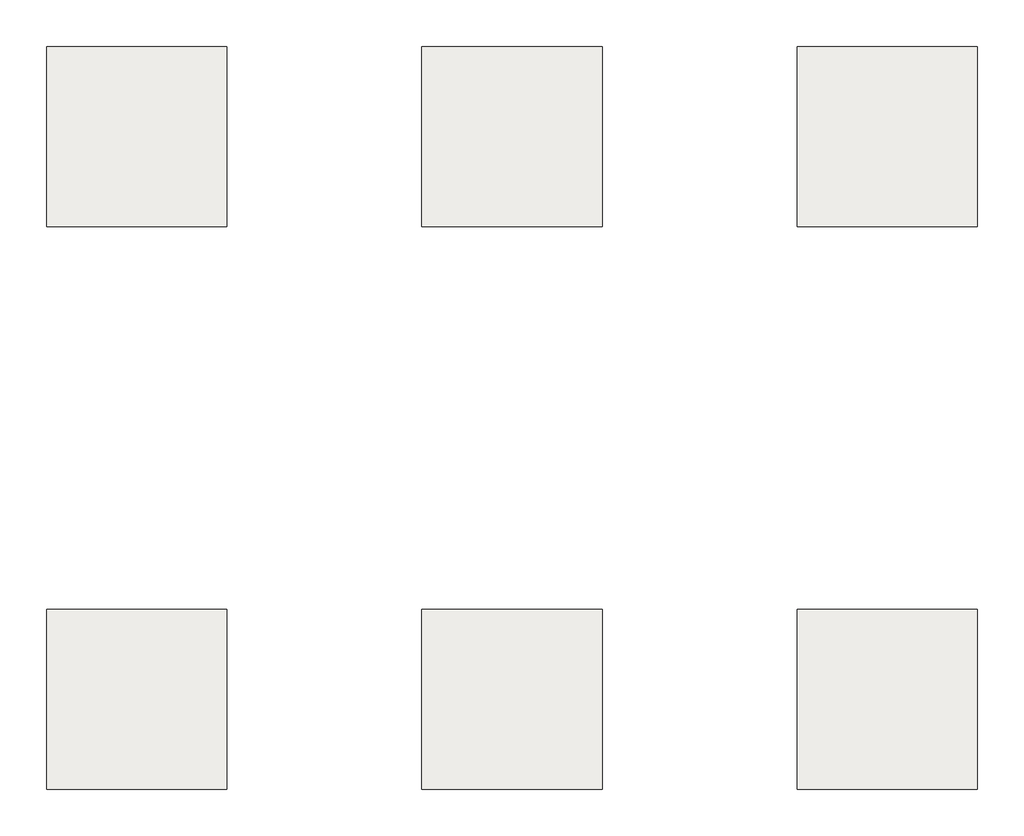
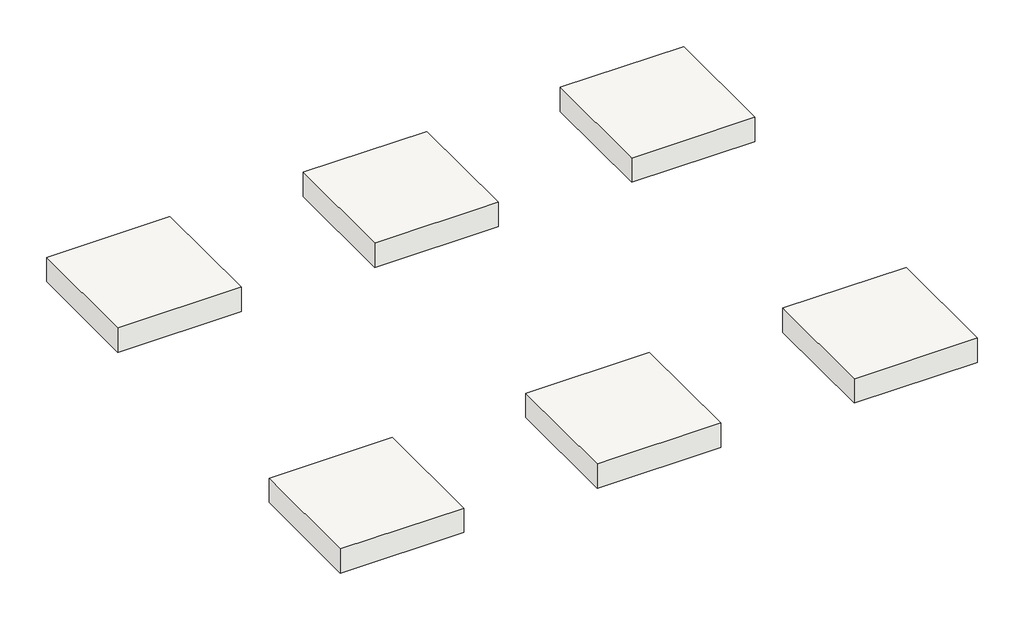
# One storey: 6 slabs.
"""IFC4 building model written with IfcOpenShell, lengths in millimetres."""

import ifcopenshell
import ifcopenshell.guid

model = None  # the IFC model being written
_history = None  # IfcOwnerHistory: only IFC2X3 demands one
_inside = {}  # id of a spatial element -> (the spatial element, [elements in it])
_under = {}  # id of a project, library or spatial element -> (it, [spatial elements below it])
_declared = {}  # id of a project -> (the project, [libraries it declares])
_typed = {}  # id of a type object -> (the type object, [elements of that type])
_made_of = {}  # id of a material, layer set ... -> (it, [elements and type objects made of it])


def new_model(schema):
    """Start an empty IFC model of exactly this schema.

    Asked for "IFC4X3", IfcOpenShell would pick the latest addendum, in which some entities
    have other attributes; the version numbers below select the first issue.
    IFC2X3 requires an IfcOwnerHistory on every rooted entity: one is made here for all.
    """
    global model, _history
    if schema == "IFC4X3":
        model = ifcopenshell.file(schema_version=(4, 3, 0, 0))
    else:
        model = ifcopenshell.file(schema=schema)
    _inside.clear()
    _under.clear()
    _declared.clear()
    _typed.clear()
    _made_of.clear()
    _history = None
    if model.schema == "IFC2X3":
        org = make("IfcOrganization", Name="unknown")
        user = make(
            "IfcPersonAndOrganization",
            ThePerson=make("IfcPerson", FamilyName="unknown"),
            TheOrganization=org,
        )
        app = make(
            "IfcApplication",
            ApplicationDeveloper=org,
            Version="unknown",
            ApplicationFullName="unknown",
            ApplicationIdentifier="unknown",
        )
        _history = make(
            "IfcOwnerHistory",
            OwningUser=user,
            OwningApplication=app,
            ChangeAction="ADDED",
            CreationDate=0,
        )
    return model


def make(cls, **values):
    """One entity of the class cls with the attributes given. An attribute that is None is left unset."""
    return model.create_entity(
        cls, **{name: value for name, value in values.items() if value is not None}
    )


def rooted(cls, **values):
    """An entity with a GlobalId (a new one), such as an element, a storey or a relation."""
    return make(cls, GlobalId=ifcopenshell.guid.new(), OwnerHistory=_history, **values)


def si_unit(unit_type, name, prefix=None):
    """IfcSIUnit, for example si_unit("LENGTHUNIT", "METRE", prefix="MILLI")."""
    return make("IfcSIUnit", UnitType=unit_type, Prefix=prefix, Name=name)


def assignment(units):
    """IfcUnitAssignment: the units of a project."""
    return None if units is None else make("IfcUnitAssignment", Units=units)


def point(xyz):
    """IfcCartesianPoint."""
    return None if xyz is None else make("IfcCartesianPoint", Coordinates=xyz)


def direction(xyz):
    """IfcDirection."""
    return None if xyz is None else make("IfcDirection", DirectionRatios=xyz)


def frame(location, z_axis=None, x_axis=None):
    """IfcAxis2Placement3D, a coordinate frame: its origin and axes. An axis left out is left unset."""
    return make(
        "IfcAxis2Placement3D",
        Location=point(location),
        Axis=direction(z_axis),
        RefDirection=direction(x_axis),
    )


def origin():
    """The frame at (0, 0, 0) with its axes left unset."""
    return frame((0.0, 0.0, 0.0))


def place(relative_to, where):
    """IfcLocalPlacement: puts the frame where relative to a parent placement (None: the world)."""
    return make(
        "IfcLocalPlacement", PlacementRelTo=relative_to, RelativePlacement=where
    )


def context(
    kind, dimensions, precision=None, world=None, true_north=None, identifier=None
):
    """IfcGeometricRepresentationContext, for example the 3D "Model" context."""
    return make(
        "IfcGeometricRepresentationContext",
        ContextIdentifier=identifier,
        ContextType=kind,
        CoordinateSpaceDimension=dimensions,
        Precision=precision,
        WorldCoordinateSystem=world,
        TrueNorth=true_north,
    )


def project(units=None, contexts=None):
    """IfcProject with its units and contexts."""
    return rooted(
        "IfcProject",
        Name="project",
        RepresentationContexts=contexts,
        UnitsInContext=assignment(units),
    )


def spatial(cls, under=None, at=None, **own):
    """A site, building, storey or space (cls), placed at a placement, below another one or the project."""
    s = rooted(cls, ObjectPlacement=at, **own)
    if under is not None:
        _under.setdefault(under.id(), (under, []))[1].append(s)
    return s


def polyline(points):
    """IfcPolyline through the points."""
    return make("IfcPolyline", Points=[point(p) for p in points])


def outline(outer, holes=None, kind="AREA"):
    """IfcArbitraryClosedProfileDef: a profile drawn as a closed curve; with holes, ...WithVoids."""
    if holes is None:
        return make("IfcArbitraryClosedProfileDef", ProfileType=kind, OuterCurve=outer)
    return make(
        "IfcArbitraryProfileDefWithVoids",
        ProfileType=kind,
        OuterCurve=outer,
        InnerCurves=holes,
    )


def extrude(swept, where, along, depth):
    """IfcExtrudedAreaSolid: the profile swept, set in the frame where, extruded along a direction by depth."""
    return make(
        "IfcExtrudedAreaSolid",
        SweptArea=swept,
        Position=where,
        ExtrudedDirection=direction(along),
        Depth=depth,
    )


def shape(context_of_items, identifier, shape_type, items):
    """IfcShapeRepresentation: the items that make up one representation, for example the "Body"."""
    return make(
        "IfcShapeRepresentation",
        ContextOfItems=context_of_items,
        RepresentationIdentifier=identifier,
        RepresentationType=shape_type,
        Items=items,
    )


def source(mapping_origin, context_of_items, identifier, shape_type, items):
    """IfcRepresentationMap: a shape defined once, which mapped items show again and again."""
    return make(
        "IfcRepresentationMap",
        MappingOrigin=mapping_origin,
        MappedRepresentation=shape(context_of_items, identifier, shape_type, items),
    )


def transform(
    local_origin,
    x_axis=None,
    y_axis=None,
    z_axis=None,
    scale=None,
    scale2=None,
    scale3=None,
    uniform=True,
):
    """IfcCartesianTransformationOperator3D, or its non-uniform kind. x_axis, y_axis, z_axis: its Axis1, 2, 3."""
    if uniform:
        return make(
            "IfcCartesianTransformationOperator3D",
            Axis1=direction(x_axis),
            Axis2=direction(y_axis),
            LocalOrigin=point(local_origin),
            Scale=scale,
            Axis3=direction(z_axis),
        )
    return make(
        "IfcCartesianTransformationOperator3DnonUniform",
        Axis1=direction(x_axis),
        Axis2=direction(y_axis),
        LocalOrigin=point(local_origin),
        Scale=scale,
        Axis3=direction(z_axis),
        Scale2=scale2,
        Scale3=scale3,
    )


def mapped(mapping_source, mapping_target):
    """IfcMappedItem: shows the shape of a source again, moved by a transform."""
    return make(
        "IfcMappedItem", MappingSource=mapping_source, MappingTarget=mapping_target
    )


def made_of(thing, what):
    """Note that an element or type object is made of a material, layer set ...; save() writes the relation."""
    if what is not None:
        _made_of.setdefault(what.id(), (what, []))[1].append(thing)
    return thing


def element(
    cls,
    number,
    at=None,
    inside=None,
    cuts=None,
    type_object=None,
    material=None,
    context=None,
    identifier="Body",
    shape_type=None,
    held_by="IfcProductDefinitionShape",
    body=None,
    shapes=None,
    **own,
):
    """One element of the class cls, such as IfcWall. Its Tag is "e" and its number.

    at: its placement. inside: the storey or other place that contains it. cuts: it is an
    opening in that element (IfcRelVoidsElement). A single representation is given by context,
    identifier, shape_type and body (its items); several are given by shapes. held_by: the class
    of the entity that holds the representations. save() writes the other relations.
    """
    e = rooted(cls, Tag="e%d" % number, ObjectPlacement=at, **own)
    if body is not None:
        shapes = [shape(context, identifier, shape_type, body)]
    if shapes is not None:
        e.Representation = make(held_by, Representations=shapes)
    if inside is not None:
        _inside.setdefault(inside.id(), (inside, []))[1].append(e)
    if cuts is not None:
        rooted(
            "IfcRelVoidsElement", RelatingBuildingElement=cuts, RelatedOpeningElement=e
        )
    if type_object is not None:
        _typed.setdefault(type_object.id(), (type_object, []))[1].append(e)
    return made_of(e, material)


def aggregate(whole, parts):
    """IfcRelAggregates: a whole, such as a stair, and the parts it consists of."""
    return rooted("IfcRelAggregates", RelatingObject=whole, RelatedObjects=parts)


def save(model, path):
    """Write the relations noted so far, then the file.

    IfcRelAggregates (storeys below a building ...), IfcRelContainedInSpatialStructure (elements
    in a storey), IfcRelDefinesByType, IfcRelAssociatesMaterial and IfcRelDeclares: one each for
    every whole, place, type object, material and project.
    """
    for whole, parts in _under.values():
        aggregate(whole, parts)
    for where, things in _inside.values():
        rooted(
            "IfcRelContainedInSpatialStructure",
            RelatedElements=things,
            RelatingStructure=where,
        )
    for kind, things in _typed.values():
        rooted("IfcRelDefinesByType", RelatedObjects=things, RelatingType=kind)
    for what, things in _made_of.values():
        rooted("IfcRelAssociatesMaterial", RelatedObjects=things, RelatingMaterial=what)
    for by, libraries in _declared.values():
        rooted("IfcRelDeclares", RelatingContext=by, RelatedDefinitions=libraries)
    model.write(path)


def ft112_footing_rectangular_ft112_2400x2400x500_5fe39465(model_context):
    return source(origin(), model_context, "Body", "SweptSolid", [
        extrude(outline(polyline([(1200.0, 1200.0), (1200.0, -1200.0), (-1200.0, -1200.0), (-1200.0, 1200.0), (1200.0, 1200.0)])), frame((0.0, 0.0, -500.0), z_axis=(0.0, 0.0, 1.0), x_axis=(1.0, 0.0, 0.0)), (0.0, 0.0, 1.0), 500.0),
    ])


model = new_model("IFC4")

# Units and contexts
model_context = context("Model", 3, world=origin())
ifc_project = project(units=[si_unit("LENGTHUNIT", "METRE", prefix="MILLI")], contexts=[model_context])

# Site, building, storey
site = spatial("IfcSite", under=ifc_project)
building = spatial("IfcBuilding", under=site)
storey = spatial("IfcBuildingStorey", under=building, Name="B.O.F", Elevation=-1800.0)

# Slabs
placement = place(None, origin())
ft112_footing_rectangular_ft112_2400x2400x500_shape = ft112_footing_rectangular_ft112_2400x2400x500_5fe39465(model_context)
element("IfcSlab", 1, ObjectType="FT112-Footing-Rectangular : FT112_2400x2400x500", at=placement, inside=storey, context=model_context, shape_type="MappedRepresentation", body=[
    mapped(ft112_footing_rectangular_ft112_2400x2400x500_shape, transform((4920.0, 13499.5208589, -1300.0), x_axis=(1.0, 0.0, 0.0), y_axis=(0.0, 1.0, 0.0), z_axis=(0.0, 0.0, 1.0))),
])
element("IfcSlab", 2, ObjectType="FT112-Footing-Rectangular : FT112_2400x2400x500", at=placement, inside=storey, context=model_context, shape_type="MappedRepresentation", body=[
    mapped(ft112_footing_rectangular_ft112_2400x2400x500_shape, transform((9920.0, 13499.5208589, -1300.0), x_axis=(1.0, 0.0, 0.0), y_axis=(0.0, 1.0, 0.0), z_axis=(0.0, 0.0, 1.0))),
])
element("IfcSlab", 3, ObjectType="FT112-Footing-Rectangular : FT112_2400x2400x500", at=placement, inside=storey, context=model_context, shape_type="MappedRepresentation", body=[
    mapped(ft112_footing_rectangular_ft112_2400x2400x500_shape, transform((9920.0, 20999.5208589, -1300.0), x_axis=(1.0, 0.0, 0.0), y_axis=(0.0, 1.0, 0.0), z_axis=(0.0, 0.0, 1.0))),
])
element("IfcSlab", 4, ObjectType="FT112-Footing-Rectangular : FT112_2400x2400x500", at=placement, inside=storey, context=model_context, shape_type="MappedRepresentation", body=[
    mapped(ft112_footing_rectangular_ft112_2400x2400x500_shape, transform((4920.0, 20999.5208589, -1300.0), x_axis=(1.0, 0.0, 0.0), y_axis=(0.0, 1.0, 0.0), z_axis=(0.0, 0.0, 1.0))),
])
element("IfcSlab", 5, ObjectType="FT112-Footing-Rectangular : FT112_2400x2400x500", at=placement, inside=storey, context=model_context, shape_type="MappedRepresentation", body=[
    mapped(ft112_footing_rectangular_ft112_2400x2400x500_shape, transform((-80.0, 20999.5208589, -1300.0), x_axis=(1.0, 0.0, 0.0), y_axis=(0.0, 1.0, 0.0), z_axis=(0.0, 0.0, 1.0))),
])
element("IfcSlab", 6, ObjectType="FT112-Footing-Rectangular : FT112_2400x2400x500", at=placement, inside=storey, context=model_context, shape_type="MappedRepresentation", body=[
    mapped(ft112_footing_rectangular_ft112_2400x2400x500_shape, transform((-80.0, 13499.5208589, -1300.0), x_axis=(1.0, 0.0, 0.0), y_axis=(0.0, 1.0, 0.0), z_axis=(0.0, 0.0, 1.0))),
])

save(model, "model.ifc")

# Revit data of these elements
# Project information
#   Building Name = "MAIN GATE SECURITY BUILDING"
#   Project Status = "Project Status"
#   Client Name = "현대엔지니어링"
#   Project Address = "서울시 종로구 율곡로 75(계동)"
#   Project Name = "Therma Visayas Energy Project"
#   Project Number = "-"
# Grids (mm)
#   "B": line (5000, 25626.165) -> (5000, 10142.075)
#   "C": line (10000, 25626.165) -> (10000, 10142.075)
#   "A": line (0, 25626.165) -> (0, 10142.075)
#   "1": line (-4230.565, 13499.521) -> (12441.468, 13499.521)
#   "2": line (-4265.133, 20999.521) -> (12441.468, 20999.521)
# Type "FT112-Footing-Rectangular : FT112_2400x2400x500"
#   Description = "UG Shallow Foundation"
#   Width = 2400 mm
#   Length = 2400 mm
#   Foundation Thickness = 500 mm
#   hec_material3 [instance default] = none
#   hec_material2 [instance default] = A03AE056-00001_Bitumen/Bituminous/Asphalt Coating
#   hec_material1 [instance default] = A03AC035-00001_Form Work (3 times in use)_Flat
#   Structural Material [instance default] = A03AC032-00007_Structural Concrete_Type1_25MPa-30Mpa
#   Assembly Code = ""
# Elements 1, 2, 3, 4, 6 (IfcSlab, "FT112-Footing-Rectangular : FT112_2400x2400x500")
#   Comments = ""
#   F01) Building Name = "Main Gate House"
#   F11) Project Building Tag_Type-1 = "Common"
#   F12) Project Building Tag_Type-2 = "Common"
#   F13) Project Facility Code = "Facility Code"
#   F21) Structural Type = "Concrete"
#   F31) Standard Building Code = "IBC"
#   F41) Discipline = "AR"
#   F51) Plan Start Date-Engineering = "2015-01-01"
#   F52) Plan Finish Date-Engineering = "2015-12-31"
#   F53) Duration = "365"
#   F54) Actual Start Date-Engineering = "2015-01-01"
#   F55) Actual Finish Date-Engineering = "2015-12-31"
#   F61) Plan Start Date-Construction = "2016-08-19"
#   F62) Plan Finish Date-Construction = "2017-01-31"
#   F64) Actual Start Date-Construction = "2016-08-19"
#   F63) Duration = "202"
#   F65) Actual Finish Date-Construction = "2017-01-31"
#   F91) Plant Type = "CFPP"
#   F92) KKS Structures, Building = "UYF"
#   P01) Project Name = "TVEP"
#   P02) Project Configuration = "CFB Boiler x 2(Foster Wheeler) + STG x 2(Alstom, 150MW)"
#   P03) Project Abbreviation = "TVEP"
#   P04) Project Code = "BEPH1402"
#   P05) Project Stage = "In operation"
#   P06) Project Location = "Sito Looc, Barangay Bato, Toledo City in Philippines"
#   P07) Project Owner = "Therma Visayas, Inc."
#   P08) Project O.E = "Flour"
#   P09) Project Schedule = "ITB Issueing Date : 2013.07.30\r\nSite Survey : 2013.08.19-20\r\nBid Closing Date : 2013.11.29\r\nPreferred Bidder Notice 접수 : 2014.04.27\r\nTarget award date : 2014 05\r\nLOA 접수 : 2014.05.21\r\nSigning Ceremony : 2014.05.30"
#   P10) Basic Wind Speed = "55.6 m/s"
#   P11) Seismic = "NSCP 2010, Zone 4 (PGA : 0.4g)"
#   P12) Soil = "Sc"
#   P13) Soil Capacity = "100kN/m2"
#   P14) Pile Capacity = "PHC(D400) : 1200kN"
#   W00) Work Master Code = "A03AC032-00007"
#   W01) Work Master_Lv1 = "Concrete Work"
#   W02) Work Master_Lv2 = "Substructure Work"
#   W03) Work Master_Spec.1 = "Cement Type-1"
#   W04) Work Master_Spec.2 = "25MPa < F'c (Cylinder Strength) ≤ 30MPa"
#   W11) Activity ID = "C02AGB010"
#   W12) Activity Name = "Main Gate Security Building - Building Foundation"
#   W13) Plan Start Date = "2016-08-19"
#   W14) Plan Finish Date = "2016-09-22"
#   W15) Duration = "26"
#   W16) Actual Start Date = "2016-08-19"
#   W17) Actual Finish Date = "2016-09-22"
#   R02) Unit Price = 0
#   Structural Material = A03AD032-00007_Structural Concrete_25MPa-30MPa
#   hec_material3 = none
#   hec_material2 = none
#   hec_material1 = none
#   Phase Created = New Construction
#   Materials on its faces: "A03AD032-00007_Structural Concrete_25MPa-30MPa"
# Element 5 (IfcSlab, "FT112-Footing-Rectangular : FT112_2400x2400x500")
#   Comments = ""
#   F01) Building Name = "Main Gate House"
#   F11) Project Building Tag_Type-1 = "Common"
#   F12) Project Building Tag_Type-2 = "Common"
#   F13) Project Facility Code = "Facility Code"
#   F21) Structural Type = "Concrete"
#   F31) Standard Building Code = "IBC"
#   F41) Discipline = "AR"
#   F51) Plan Start Date-Engineering = "2015-01-01"
#   F52) Plan Finish Date-Engineering = "2015-12-31"
#   F53) Duration = "365"
#   F54) Actual Start Date-Engineering = "2015-01-01"
#   F55) Actual Finish Date-Engineering = "2015-12-31"
#   F61) Plan Start Date-Construction = "2016-08-19"
#   F62) Plan Finish Date-Construction = "2017-01-31"
#   F64) Actual Start Date-Construction = "2016-08-19"
#   F63) Duration = "202"
#   F65) Actual Finish Date-Construction = "2017-01-31"
#   F91) Plant Type = "CFPP"
#   F92) KKS Structures, Building = "UYF"
#   P01) Project Name = "TVEP"
#   P02) Project Configuration = "CFB Boiler x 2(Foster Wheeler) + STG x 2(Alstom, 150MW)"
#   P03) Project Abbreviation = "TVEP"
#   P04) Project Code = "BEPH1402"
#   P05) Project Stage = "In operation"
#   P06) Project Location = "Sito Looc, Barangay Bato, Toledo City in Philippines"
#   P07) Project Owner = "Therma Visayas, Inc."
#   P08) Project O.E = "Flour"
#   P09) Project Schedule = "ITB Issueing Date : 2013.07.30\r\nSite Survey : 2013.08.19-20\r\nBid Closing Date : 2013.11.29\r\nPreferred Bidder Notice 접수 : 2014.04.27\r\nTarget award date : 2014 05\r\nLOA 접수 : 2014.05.21\r\nSigning Ceremony : 2014.05.30"
#   P10) Basic Wind Speed = "55.6 m/s"
#   P11) Seismic = "NSCP 2010, Zone 4 (PGA : 0.4g)"
#   P12) Soil = "Sc"
#   P13) Soil Capacity = "100kN/m2"
#   P14) Pile Capacity = "PHC(D400) : 1200kN"
#   W00) Work Master Code = "A03AC032-00007"
#   W01) Work Master_Lv1 = "Concrete Work"
#   W02) Work Master_Lv2 = "Substructure Work"
#   W03) Work Master_Spec.1 = "Cement Type-1"
#   W04) Work Master_Spec.2 = "25MPa < F'c (Cylinder Strength) ≤ 30MPa"
#   W11) Activity ID = "C02AGB010"
#   W12) Activity Name = "Main Gate Security Building - Building Foundation"
#   W13) Plan Start Date = "2016-08-19"
#   W14) Plan Finish Date = "2016-09-22"
#   W15) Duration = "26"
#   W16) Actual Start Date = "2016-08-19"
#   W17) Actual Finish Date = "2016-09-22"
#   R02) Unit Price = 0
#   Structural Material = A03AD032-00007_Structural Concrete_25MPa-30MPa
#   hec_material3 = none
#   hec_material2 = none
#   hec_material1 = A03AD035-2505_Form Work_3 times
#   Phase Created = New Construction
#   Materials on its faces: "A03AD032-00007_Structural Concrete_25MPa-30MPa"
# Materials
#   "A03AE056-00001_Bitumen/Bituminous/Asphalt Coating": class "Generic", colour RGB 17 17 17, transparency 0, Description = "Damp-proofing", W00) Work Master Code = "A03AE056-00001", W01) Work Master_Lv1 = "Concrete Work", W02) Work Master_Lv2 = "Concrete Protective Coating (U/G)", W03) Work Master_Spec.1 = "Bitumen/Bituminous/Asphalt Coating", Cost = 0
#   "A03AC035-00001_Form Work (3 times in use)_Flat": class "Wood", colour RGB 149 120 74, transparency 0, Description = "Plywood", W00) Work Master Code = "A03AC035-00001", W01) Work Master_Lv1 = "Concrete Work", W02) Work Master_Lv2 = "Substructure Work", W03) Work Master_Spec.1 = "Form Work (3 times in use)", W04) Work Master_Spec.2 = "Flat Form", W05) Work Master_Spec.3 = "Dressed Lumber, Plywood or Steel Form(Wood Planks are not Allowed) incl. Chamfer", Cost = 0
#   "A03AC032-00007_Structural Concrete_Type1_25MPa-30Mpa": class "Concrete", colour RGB 176 176 176, transparency 0, Keynote = "09910.A1", Description = "Reinf. Conc.", W00) Work Master Code = "A03AC032-00007", W01) Work Master_Lv1 = "Concrete Work", W02) Work Master_Lv2 = "Substructure Work", W03) Work Master_Spec.1 = "Structural Concrete", W04) Work Master_Spec.2 = "Cement Type-1", W05) Work Master_Spec.3 = "25MPa < F'c (Cylinder Strength) ≤ 30MPa", Cost = 0
#   "A03AD032-00007_Structural Concrete_25MPa-30MPa": class "Concrete", colour RGB 176 176 176, transparency 0, Keynote = "09910.A1", Description = "Reinf. Conc.", W00) Work Master Code = "A03AD032-00007", W01) Work Master_Lv1 = "Concrete Work", W02) Work Master_Lv2 = "Superstructure Work", W03) Work Master_Spec.1 = "Structural Concrete", W04) Work Master_Spec.2 = "Cement Type-1", W05) Work Master_Spec.3 = "25MPa < F'c (Cylinder Strength) ≤ 30MPa", Cost = 0
#   "A03AD035-2505_Form Work_3 times": class "Wood", colour RGB 149 120 74, transparency 0, Description = "Plywood", W00) Work Master Code = "A03AD035-2505", W01) Work Master_Lv1 = "Concrete Work", W02) Work Master_Lv2 = "Superstructure Work", W03) Work Master_Spec.1 = "Form Work (3 times in use)", W04) Work Master_Spec.2 = "Flat Form", W05) Work Master_Spec.3 = "Dressed Lumber, Plywood or Steel Form(Wood Planks are not Allowed) incl. Chamfer", Cost = 0
